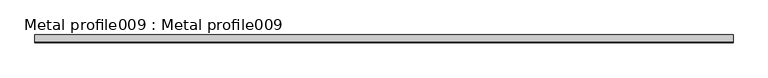
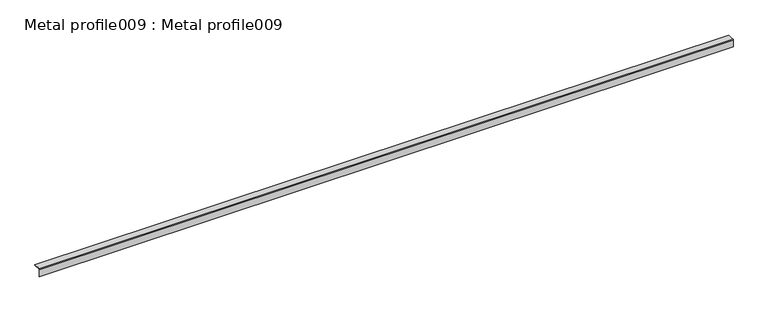
"""IFC4 building model written with IfcOpenShell, lengths in millimetres: proxy geometry, Metal profile009 : Metal profile009."""

import ifcopenshell
import ifcopenshell.guid

model = None  # the IFC model being written
_history = None  # IfcOwnerHistory: only IFC2X3 demands one
_inside = {}  # id of a spatial element -> (the spatial element, [elements in it])
_under = {}  # id of a project, library or spatial element -> (it, [spatial elements below it])
_declared = {}  # id of a project -> (the project, [libraries it declares])
_typed = {}  # id of a type object -> (the type object, [elements of that type])
_made_of = {}  # id of a material, layer set ... -> (it, [elements and type objects made of it])


def new_model(schema):
    """Start an empty IFC model of exactly this schema.

    Asked for "IFC4X3", IfcOpenShell would pick the latest addendum, in which some entities
    have other attributes; the version numbers below select the first issue.
    IFC2X3 requires an IfcOwnerHistory on every rooted entity: one is made here for all.
    """
    global model, _history
    if schema == "IFC4X3":
        model = ifcopenshell.file(schema_version=(4, 3, 0, 0))
    else:
        model = ifcopenshell.file(schema=schema)
    _inside.clear()
    _under.clear()
    _declared.clear()
    _typed.clear()
    _made_of.clear()
    _history = None
    if model.schema == "IFC2X3":
        org = make("IfcOrganization", Name="unknown")
        user = make(
            "IfcPersonAndOrganization",
            ThePerson=make("IfcPerson", FamilyName="unknown"),
            TheOrganization=org,
        )
        app = make(
            "IfcApplication",
            ApplicationDeveloper=org,
            Version="unknown",
            ApplicationFullName="unknown",
            ApplicationIdentifier="unknown",
        )
        _history = make(
            "IfcOwnerHistory",
            OwningUser=user,
            OwningApplication=app,
            ChangeAction="ADDED",
            CreationDate=0,
        )
    return model


def make(cls, **values):
    """One entity of the class cls with the attributes given. An attribute that is None is left unset."""
    return model.create_entity(
        cls, **{name: value for name, value in values.items() if value is not None}
    )


def rooted(cls, **values):
    """An entity with a GlobalId (a new one), such as an element, a storey or a relation."""
    return make(cls, GlobalId=ifcopenshell.guid.new(), OwnerHistory=_history, **values)


def si_unit(unit_type, name, prefix=None):
    """IfcSIUnit, for example si_unit("LENGTHUNIT", "METRE", prefix="MILLI")."""
    return make("IfcSIUnit", UnitType=unit_type, Prefix=prefix, Name=name)


def assignment(units):
    """IfcUnitAssignment: the units of a project."""
    return None if units is None else make("IfcUnitAssignment", Units=units)


def point(xyz):
    """IfcCartesianPoint."""
    return None if xyz is None else make("IfcCartesianPoint", Coordinates=xyz)


def direction(xyz):
    """IfcDirection."""
    return None if xyz is None else make("IfcDirection", DirectionRatios=xyz)


def frame(location, z_axis=None, x_axis=None):
    """IfcAxis2Placement3D, a coordinate frame: its origin and axes. An axis left out is left unset."""
    return make(
        "IfcAxis2Placement3D",
        Location=point(location),
        Axis=direction(z_axis),
        RefDirection=direction(x_axis),
    )


def frame_2d(location, x_axis=None):
    """IfcAxis2Placement2D, a coordinate frame in the plane: its origin and x axis."""
    return make(
        "IfcAxis2Placement2D", Location=point(location), RefDirection=direction(x_axis)
    )


def origin():
    """The frame at (0, 0, 0) with its axes left unset."""
    return frame((0.0, 0.0, 0.0))


def place(relative_to, where):
    """IfcLocalPlacement: puts the frame where relative to a parent placement (None: the world)."""
    return make(
        "IfcLocalPlacement", PlacementRelTo=relative_to, RelativePlacement=where
    )


def context(
    kind, dimensions, precision=None, world=None, true_north=None, identifier=None
):
    """IfcGeometricRepresentationContext, for example the 3D "Model" context."""
    return make(
        "IfcGeometricRepresentationContext",
        ContextIdentifier=identifier,
        ContextType=kind,
        CoordinateSpaceDimension=dimensions,
        Precision=precision,
        WorldCoordinateSystem=world,
        TrueNorth=true_north,
    )


def project(units=None, contexts=None):
    """IfcProject with its units and contexts."""
    return rooted(
        "IfcProject",
        Name="project",
        RepresentationContexts=contexts,
        UnitsInContext=assignment(units),
    )


def spatial(cls, under=None, at=None, **own):
    """A site, building, storey or space (cls), placed at a placement, below another one or the project."""
    s = rooted(cls, ObjectPlacement=at, **own)
    if under is not None:
        _under.setdefault(under.id(), (under, []))[1].append(s)
    return s


def polyline(points):
    """IfcPolyline through the points."""
    return make("IfcPolyline", Points=[point(p) for p in points])


def circle_curve(where, radius):
    """IfcCircle in the frame where."""
    return make("IfcCircle", Position=where, Radius=radius)


def trimmed(basis, trim1, trim2, sense, master):
    """IfcTrimmedCurve: the piece of a basis curve between two trims."""
    return make(
        "IfcTrimmedCurve",
        BasisCurve=basis,
        Trim1=trim1,
        Trim2=trim2,
        SenseAgreement=sense,
        MasterRepresentation=master,
    )


def segment(curve, same_sense, transition):
    """IfcCompositeCurveSegment."""
    return make(
        "IfcCompositeCurveSegment",
        Transition=transition,
        SameSense=same_sense,
        ParentCurve=curve,
    )


def composite_curve(segments, self_intersect=None):
    """IfcCompositeCurve: segments joined end to end."""
    return make("IfcCompositeCurve", Segments=segments, SelfIntersect=self_intersect)


def outline(outer, holes=None, kind="AREA"):
    """IfcArbitraryClosedProfileDef: a profile drawn as a closed curve; with holes, ...WithVoids."""
    if holes is None:
        return make("IfcArbitraryClosedProfileDef", ProfileType=kind, OuterCurve=outer)
    return make(
        "IfcArbitraryProfileDefWithVoids",
        ProfileType=kind,
        OuterCurve=outer,
        InnerCurves=holes,
    )


def extrude(swept, where, along, depth):
    """IfcExtrudedAreaSolid: the profile swept, set in the frame where, extruded along a direction by depth."""
    return make(
        "IfcExtrudedAreaSolid",
        SweptArea=swept,
        Position=where,
        ExtrudedDirection=direction(along),
        Depth=depth,
    )


def shape(context_of_items, identifier, shape_type, items):
    """IfcShapeRepresentation: the items that make up one representation, for example the "Body"."""
    return make(
        "IfcShapeRepresentation",
        ContextOfItems=context_of_items,
        RepresentationIdentifier=identifier,
        RepresentationType=shape_type,
        Items=items,
    )


def source(mapping_origin, context_of_items, identifier, shape_type, items):
    """IfcRepresentationMap: a shape defined once, which mapped items show again and again."""
    return make(
        "IfcRepresentationMap",
        MappingOrigin=mapping_origin,
        MappedRepresentation=shape(context_of_items, identifier, shape_type, items),
    )


def transform(
    local_origin,
    x_axis=None,
    y_axis=None,
    z_axis=None,
    scale=None,
    scale2=None,
    scale3=None,
    uniform=True,
):
    """IfcCartesianTransformationOperator3D, or its non-uniform kind. x_axis, y_axis, z_axis: its Axis1, 2, 3."""
    if uniform:
        return make(
            "IfcCartesianTransformationOperator3D",
            Axis1=direction(x_axis),
            Axis2=direction(y_axis),
            LocalOrigin=point(local_origin),
            Scale=scale,
            Axis3=direction(z_axis),
        )
    return make(
        "IfcCartesianTransformationOperator3DnonUniform",
        Axis1=direction(x_axis),
        Axis2=direction(y_axis),
        LocalOrigin=point(local_origin),
        Scale=scale,
        Axis3=direction(z_axis),
        Scale2=scale2,
        Scale3=scale3,
    )


def mapped(mapping_source, mapping_target):
    """IfcMappedItem: shows the shape of a source again, moved by a transform."""
    return make(
        "IfcMappedItem", MappingSource=mapping_source, MappingTarget=mapping_target
    )


def made_of(thing, what):
    """Note that an element or type object is made of a material, layer set ...; save() writes the relation."""
    if what is not None:
        _made_of.setdefault(what.id(), (what, []))[1].append(thing)
    return thing


def element(
    cls,
    number,
    at=None,
    inside=None,
    cuts=None,
    type_object=None,
    material=None,
    context=None,
    identifier="Body",
    shape_type=None,
    held_by="IfcProductDefinitionShape",
    body=None,
    shapes=None,
    **own,
):
    """One element of the class cls, such as IfcWall. Its Tag is "e" and its number.

    at: its placement. inside: the storey or other place that contains it. cuts: it is an
    opening in that element (IfcRelVoidsElement). A single representation is given by context,
    identifier, shape_type and body (its items); several are given by shapes. held_by: the class
    of the entity that holds the representations. save() writes the other relations.
    """
    e = rooted(cls, Tag="e%d" % number, ObjectPlacement=at, **own)
    if body is not None:
        shapes = [shape(context, identifier, shape_type, body)]
    if shapes is not None:
        e.Representation = make(held_by, Representations=shapes)
    if inside is not None:
        _inside.setdefault(inside.id(), (inside, []))[1].append(e)
    if cuts is not None:
        rooted(
            "IfcRelVoidsElement", RelatingBuildingElement=cuts, RelatedOpeningElement=e
        )
    if type_object is not None:
        _typed.setdefault(type_object.id(), (type_object, []))[1].append(e)
    return made_of(e, material)


def aggregate(whole, parts):
    """IfcRelAggregates: a whole, such as a stair, and the parts it consists of."""
    return rooted("IfcRelAggregates", RelatingObject=whole, RelatedObjects=parts)


def save(model, path):
    """Write the relations noted so far, then the file.

    IfcRelAggregates (storeys below a building ...), IfcRelContainedInSpatialStructure (elements
    in a storey), IfcRelDefinesByType, IfcRelAssociatesMaterial and IfcRelDeclares: one each for
    every whole, place, type object, material and project.
    """
    for whole, parts in _under.values():
        aggregate(whole, parts)
    for where, things in _inside.values():
        rooted(
            "IfcRelContainedInSpatialStructure",
            RelatedElements=things,
            RelatingStructure=where,
        )
    for kind, things in _typed.values():
        rooted("IfcRelDefinesByType", RelatedObjects=things, RelatingType=kind)
    for what, things in _made_of.values():
        rooted("IfcRelAssociatesMaterial", RelatedObjects=things, RelatingMaterial=what)
    for by, libraries in _declared.values():
        rooted("IfcRelDeclares", RelatingContext=by, RelatedDefinitions=libraries)
    model.write(path)


def metal_profile009_metal_profile009_1b92bf4f(model_context):
    return source(origin(), model_context, "Body", "SweptSolid", [
        extrude(outline(composite_curve([segment(polyline([(10284.5464235, 40794.44275), (10263.3932396, 40794.44275), (10263.3932396, 40773.2895661), (10262.1132396, 40773.2895661), (10262.1132396, 40794.1924758)]), True, "CONTINUOUS"), segment(trimmed(circle_curve(frame_2d((10262.7532396, 40795.08275)), 1.0964434), [point((10262.1132396, 40794.1924758))], [point((10263.6435138, 40795.72275))], False, "CARTESIAN"), True, "CONTINUOUS"), segment(polyline([(10263.6435138, 40795.72275), (10284.5464235, 40795.72275), (10284.5464235, 40794.44275)]), True, "CONTINUOUS")], self_intersect=False)), frame((3694.2883192, 0.0, 0.0), z_axis=(1.0, 0.0, 0.0), x_axis=(0.0, 1.0, 0.0)), (0.0, 0.0, 1.0), 2000.0),
    ])


if __name__ == "__main__":
    model = new_model("IFC4")
    model_context = context("Model", 3, world=origin())
    ifc_project = project(units=[si_unit("LENGTHUNIT", "METRE", prefix="MILLI")], contexts=[model_context])
    site = spatial("IfcSite", under=ifc_project)
    building = spatial("IfcBuilding", under=site)
    placement = place(None, origin())
    metal_profile009_metal_profile009_shape = metal_profile009_metal_profile009_1b92bf4f(model_context)
    element("IfcBuildingElementProxy", 1, Name="Metal profile009 : Metal profile009", ObjectType="Metal profile009 : Metal profile009", at=placement, inside=building, context=model_context, shape_type="MappedRepresentation", body=[
        mapped(metal_profile009_metal_profile009_shape, transform((0.0, 0.0, 0.0), x_axis=(1.0, 0.0, 0.0), y_axis=(0.0, 1.0, 0.0), z_axis=(0.0, 0.0, 1.0))),
    ])
    save(model, "model.ifc")

# Revit data of these elements
# Type "Metal profile009 : Metal profile009"
#   NameOverride = "Metal profile009"
# Element 1 (IfcBuildingElementProxy, "Metal profile009 : Metal profile009")
#   Materials on its faces: "CORNER BEAD"
# Materials
#   "CORNER BEAD": class "Unassigned", colour RGB 253 236 176, transparency 0, Cost = 0
